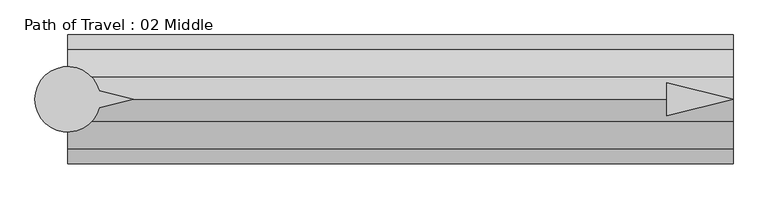
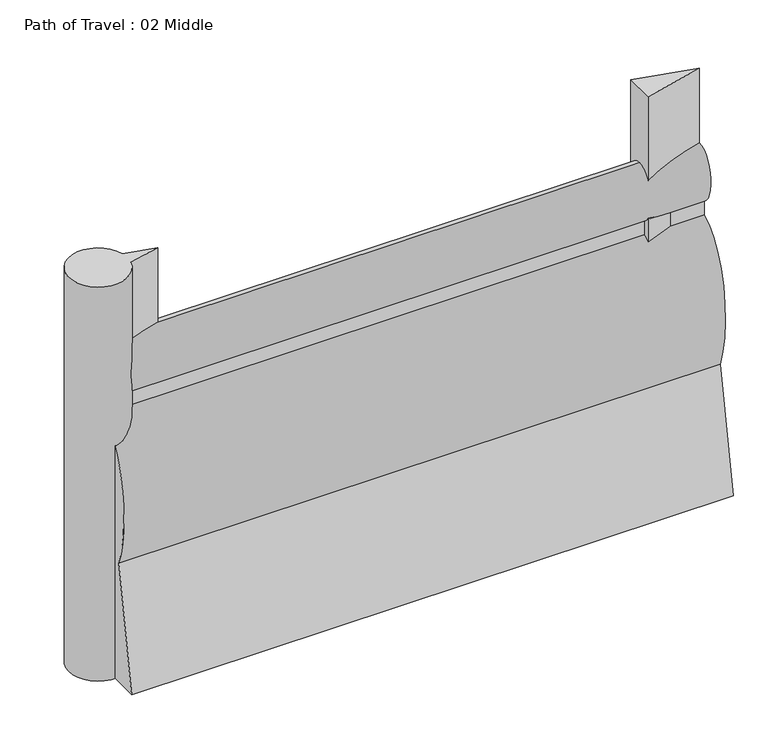
"""IFC4 building model written with IfcOpenShell, lengths in millimetres: proxy geometry, Path of Travel : 02 Middle."""

from ifc_helpers import new_model, si_unit, point, frame, frame_2d, origin, origin_with_axes, place, context, project, spatial, polyline, circle_curve, ellipse_curve, trimmed, segment, composite_curve, outline, extrude, source, transform, mapped, element, save
from ifc_brep_helpers import plane_surface, extruded_surface, advanced_brep


def path_of_travel_02_middle_b2226c54(model_context):
    return source(origin(), model_context, "Body", "SolidModel", [
        advanced_brep(
        [(227.5554837, 0.0, 1727.2), (227.5554837, 42.9018657, 1436.6534209), (227.5554837, 42.9018657, 1363.4763406), (227.5554837, 184.1186263, 643.4144547), (227.5554837, 297.5699544, 0.0), (227.5554837, 145.6574193, 0.0), (227.5554837, 0.0, 584.2), (227.5554837, -145.6574193, 0.0), (227.5554837, -297.5699544, 0.0), (227.5554837, -184.1186263, 643.4144547), (227.5554837, -42.9018657, 1363.4763406), (227.5554837, -42.9018657, 1436.6534209), (3300.9554837, 0.0, 1727.2), (3300.9554837, -42.9018657, 1436.6534209), (3300.9554837, -42.9018657, 1363.4763406), (3300.9554837, -184.1186263, 643.4144547), (3300.9554837, -297.5699544, 0.0), (3300.9554837, -145.6574193, 0.0), (3300.9554837, 0.0, 584.2), (3300.9554837, 145.6574193, 0.0), (3300.9554837, 297.5699544, 0.0), (3300.9554837, 184.1186263, 643.4144547), (3300.9554837, 42.9018657, 1363.4763406), (3300.9554837, 42.9018657, 1436.6534209)],
        [
            (0, 1, ellipse_curve(frame((227.5554837, 0.0, 1574.8), z_axis=(-1.0, 0.0, 0.0), x_axis=(0.0, 0.0, 1.0)), 152.4, 101.6)),
            (1, 2),
            (2, 3, ellipse_curve(frame((227.5554837, 0.0, 914.4), z_axis=(-1.0, 0.0, 0.0), x_axis=(0.0, 0.0, -1.0)), 457.2, 228.6)),
            (3, 4),
            (4, 5),
            (5, 6),
            (6, 7),
            (7, 8),
            (8, 9),
            (9, 10, ellipse_curve(frame((227.5554837, 0.0, 914.4), z_axis=(-1.0, 0.0, 0.0), x_axis=(0.0, 0.0, -1.0)), 457.2, 228.6)),
            (10, 11),
            (11, 0, ellipse_curve(frame((227.5554837, 0.0, 1574.8), z_axis=(-1.0, 0.0, 0.0), x_axis=(0.0, 0.0, 1.0)), 152.4, 101.6)),
            (12, 13, ellipse_curve(frame((3300.9554837, 0.0, 1574.8), z_axis=(1.0, 0.0, 0.0), x_axis=(0.0, 0.0, 1.0)), 152.4, 101.6)),
            (13, 14),
            (14, 15, ellipse_curve(frame((3300.9554837, 0.0, 914.4), z_axis=(1.0, 0.0, 0.0), x_axis=(0.0, 0.0, -1.0)), 457.2, 228.6)),
            (15, 16),
            (16, 17),
            (17, 18),
            (18, 19),
            (19, 20),
            (20, 21),
            (21, 22, ellipse_curve(frame((3300.9554837, 0.0, 914.4), z_axis=(1.0, 0.0, 0.0), x_axis=(0.0, 0.0, -1.0)), 457.2, 228.6)),
            (22, 23),
            (23, 12, ellipse_curve(frame((3300.9554837, 0.0, 1574.8), z_axis=(1.0, 0.0, 0.0), x_axis=(0.0, 0.0, 1.0)), 152.4, 101.6)),
            (0, 12),
            (23, 1),
            (22, 2),
            (21, 3),
            (20, 4),
            (19, 5),
            (18, 6),
            (17, 7),
            (16, 8),
            (15, 9),
            (14, 10),
            (13, 11),
        ],
        [
            plane_surface(frame((227.5554837, 0.0, 0.0), z_axis=(-1.0, 0.0, 0.0), x_axis=(0.0, 0.0, 1.0))),
            plane_surface(frame((3300.9554837, 0.0, 0.0), z_axis=(1.0, 0.0, 0.0), x_axis=(0.0, 0.0, 1.0))),
            extruded_surface(trimmed(ellipse_curve(frame((3300.9554837, 0.0, 1574.8), z_axis=(-1.0, 0.0, 0.0), x_axis=(0.0, 0.0, 1.0)), 152.4, 101.6), [point((3300.9554837, 0.0, 1727.2))], [point((3300.9554837, 42.9018657, 1436.6534209))], True, "CARTESIAN"), (-3073.4, 0.0, 0.0), 3073.4),
            plane_surface(frame((227.5554837, 42.9018657, 1436.6534209), z_axis=(0.0, 1.0, 0.0), x_axis=(1.0, 0.0, 0.0))),
            extruded_surface(trimmed(ellipse_curve(frame((3300.9554837, 0.0, 914.4), z_axis=(-1.0, 0.0, 0.0), x_axis=(0.0, 0.0, -1.0)), 457.2, 228.6), [point((3300.9554837, 42.9018657, 1363.4763406))], [point((3300.9554837, 184.1186263, 643.4144547))], True, "CARTESIAN"), (-3073.4, 0.0, 0.0), 3073.4),
            plane_surface(frame((227.5554837, 184.1186263, 643.4144547), z_axis=(0.0, 0.9848077530122078, 0.1736481776669322), x_axis=(1.0, 0.0, 0.0))),
            plane_surface(frame((227.5554837, 297.5699544, 0.0), z_axis=(0.0, 0.0, -1.0), x_axis=(1.0, 0.0, 0.0))),
            plane_surface(frame((227.5554837, 145.6574193, 0.0), z_axis=(0.0, -0.9702957262760199, -0.2419218955995739), x_axis=(1.0, 0.0, 0.0))),
            plane_surface(frame((227.5554837, 0.0, 584.2), z_axis=(0.0, 0.9702957262759961, -0.24192189559966923), x_axis=(1.0, 0.0, 0.0))),
            plane_surface(frame((227.5554837, -145.6574193, 0.0), z_axis=(0.0, 0.0, -1.0), x_axis=(1.0, 0.0, 0.0))),
            plane_surface(frame((227.5554837, -297.5699544, 0.0), z_axis=(0.0, -0.984807753012208, 0.17364817766693066), x_axis=(1.0, 0.0, 0.0))),
            extruded_surface(trimmed(ellipse_curve(frame((3300.9554837, 0.0, 914.4), z_axis=(-1.0, 0.0, 0.0), x_axis=(0.0, 0.0, -1.0)), 457.2, 228.6), [point((3300.9554837, -184.1186263, 643.4144547))], [point((3300.9554837, -42.9018657, 1363.4763406))], True, "CARTESIAN"), (-3073.4, 0.0, 0.0), 3073.4),
            plane_surface(frame((227.5554837, -42.9018657, 1363.4763406), z_axis=(0.0, -1.0, 0.0), x_axis=(1.0, 0.0, 0.0))),
            extruded_surface(trimmed(ellipse_curve(frame((3300.9554837, 0.0, 1574.8), z_axis=(-1.0, 0.0, 0.0), x_axis=(0.0, 0.0, 1.0)), 152.4, 101.6), [point((3300.9554837, -42.9018657, 1436.6534209))], [point((3300.9554837, 0.0, 1727.2))], True, "CARTESIAN"), (-3073.4, 0.0, 0.0), 3073.4),
        ],
        [
            (0, [[1, 2, 3, 4, 5, 6, 7, 8, 9, 10, 11, 12]]),
            (1, [[13, 14, 15, 16, 17, 18, 19, 20, 21, 22, 23, 24]]),
            (2, [[-1, 25, -24, 26]]),
            (3, [[-2, -26, -23, 27]]),
            (4, [[-3, -27, -22, 28]]),
            (5, [[-4, -28, -21, 29]]),
            (6, [[-5, -29, -20, 30]]),
            (7, [[-6, -30, -19, 31]]),
            (8, [[-7, -31, -18, 32]]),
            (9, [[-8, -32, -17, 33]]),
            (10, [[-9, -33, -16, 34]]),
            (11, [[-10, -34, -15, 35]]),
            (12, [[-11, -35, -14, 36]]),
            (13, [[-12, -36, -13, -25]]),
        ],
    ),
        extrude(outline(polyline([(2994.9503371, 76.2006338), (3300.9554837, 0.0), (2994.9503371, -76.2006338), (2994.9503371, 76.2006338)])), origin_with_axes(), (0.0, 0.0, 1.0), 2129.5973753),
        extrude(outline(composite_curve([segment(polyline([(372.7837828, 39.4440225), (531.182385, 0.0), (372.7837828, -39.4440225)]), True, "CONTINUOUS"), segment(trimmed(circle_curve(frame_2d((227.2200886, 0.0)), 150.8131956), [point((372.7837828, -39.4440225))], [point((372.7837828, 39.4440225))], False, "CARTESIAN"), True, "CONTINUOUS")], self_intersect=False)), origin_with_axes(), (0.0, 0.0, 1.0), 2129.5973753),
    ])


if __name__ == "__main__":
    model = new_model("IFC4")
    model_context = context("Model", 3, world=origin())
    ifc_project = project(units=[si_unit("LENGTHUNIT", "METRE", prefix="MILLI")], contexts=[model_context])
    site = spatial("IfcSite", under=ifc_project)
    building = spatial("IfcBuilding", under=site)
    placement = place(None, origin())
    path_of_travel_02_middle_shape = path_of_travel_02_middle_b2226c54(model_context)
    element("IfcBuildingElementProxy", 1, Name="Path of Travel : 02 Middle", ObjectType="Path of Travel : 02 Middle", at=placement, inside=building, context=model_context, shape_type="MappedRepresentation", body=[
        mapped(path_of_travel_02_middle_shape, transform((0.0, 0.0, 0.0), x_axis=(1.0, 0.0, 0.0), y_axis=(0.0, 1.0, 0.0), z_axis=(0.0, 0.0, 1.0))),
    ])
    save(model, "model.ifc")

# Revit data of these elements
# Type "Path of Travel : 02 Middle"
#   Path of Egress [instance default] = 4' - 0"
#   built-in parameter 1001306 [instance default] = 4 (stored number, unit not read)
#   Dot at Start = no
#   Arrow in Middle = yes
#   Arrow at End = no
#   Egress Path = none
# Element 1 (IfcBuildingElementProxy, "Path of Travel : 02 Middle")
#   Path of Egress = 10' - 1"
#   built-in parameter 1001306 = 10.0833 (stored number, unit not read)
#   Materials on its faces: "Egress Path Solid", "solid"
# Materials
#   "Egress Path Solid": class "Unassigned", colour RGB 255 128 64, transparency 0.75, Comments = "Rendering appearance not upgraded "
#   "solid": class "Generic", colour RGB 120 120 120, transparency 0, Cost = 0
